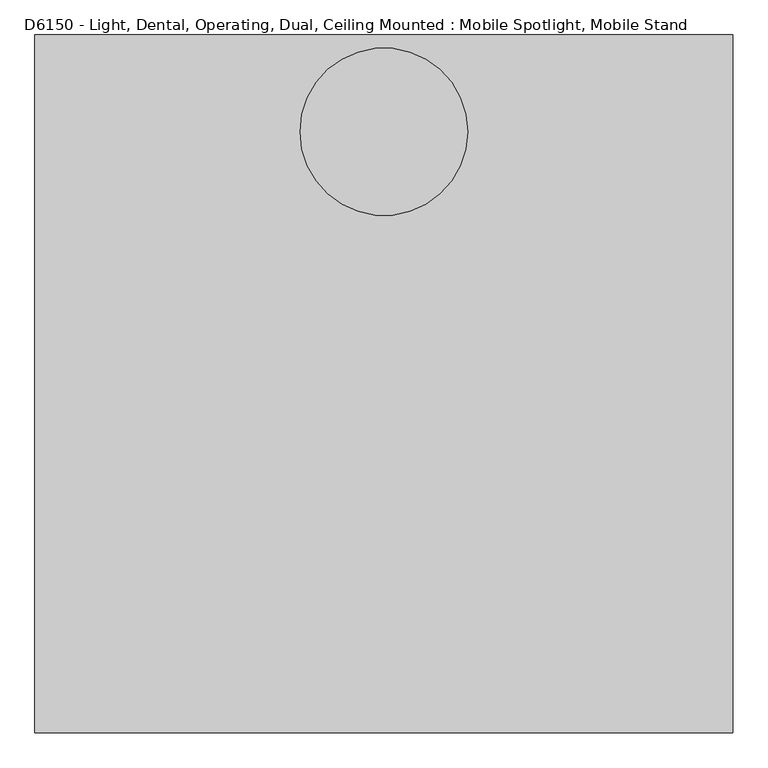
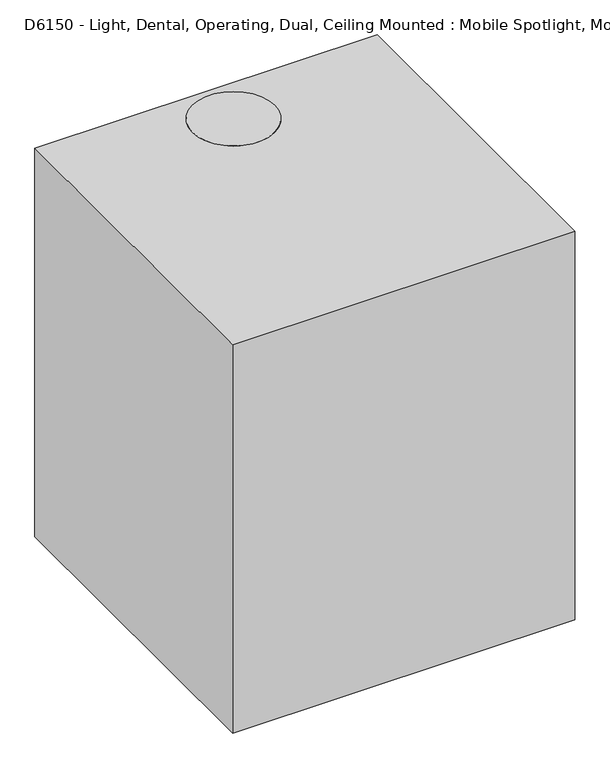
"""IFC4 building model written with IfcOpenShell, lengths in millimetres: proxy geometry, D6150 - Light, Dental, Operating, Dual, Ceiling Mounted : Mobile Spotlight, Mobile Stand."""

import ifcopenshell
import ifcopenshell.guid

model = None  # the IFC model being written
_history = None  # IfcOwnerHistory: only IFC2X3 demands one
_inside = {}  # id of a spatial element -> (the spatial element, [elements in it])
_under = {}  # id of a project, library or spatial element -> (it, [spatial elements below it])
_declared = {}  # id of a project -> (the project, [libraries it declares])
_typed = {}  # id of a type object -> (the type object, [elements of that type])
_made_of = {}  # id of a material, layer set ... -> (it, [elements and type objects made of it])


def new_model(schema):
    """Start an empty IFC model of exactly this schema.

    Asked for "IFC4X3", IfcOpenShell would pick the latest addendum, in which some entities
    have other attributes; the version numbers below select the first issue.
    IFC2X3 requires an IfcOwnerHistory on every rooted entity: one is made here for all.
    """
    global model, _history
    if schema == "IFC4X3":
        model = ifcopenshell.file(schema_version=(4, 3, 0, 0))
    else:
        model = ifcopenshell.file(schema=schema)
    _inside.clear()
    _under.clear()
    _declared.clear()
    _typed.clear()
    _made_of.clear()
    _history = None
    if model.schema == "IFC2X3":
        org = make("IfcOrganization", Name="unknown")
        user = make(
            "IfcPersonAndOrganization",
            ThePerson=make("IfcPerson", FamilyName="unknown"),
            TheOrganization=org,
        )
        app = make(
            "IfcApplication",
            ApplicationDeveloper=org,
            Version="unknown",
            ApplicationFullName="unknown",
            ApplicationIdentifier="unknown",
        )
        _history = make(
            "IfcOwnerHistory",
            OwningUser=user,
            OwningApplication=app,
            ChangeAction="ADDED",
            CreationDate=0,
        )
    return model


def make(cls, **values):
    """One entity of the class cls with the attributes given. An attribute that is None is left unset."""
    return model.create_entity(
        cls, **{name: value for name, value in values.items() if value is not None}
    )


def rooted(cls, **values):
    """An entity with a GlobalId (a new one), such as an element, a storey or a relation."""
    return make(cls, GlobalId=ifcopenshell.guid.new(), OwnerHistory=_history, **values)


def si_unit(unit_type, name, prefix=None):
    """IfcSIUnit, for example si_unit("LENGTHUNIT", "METRE", prefix="MILLI")."""
    return make("IfcSIUnit", UnitType=unit_type, Prefix=prefix, Name=name)


def assignment(units):
    """IfcUnitAssignment: the units of a project."""
    return None if units is None else make("IfcUnitAssignment", Units=units)


def point(xyz):
    """IfcCartesianPoint."""
    return None if xyz is None else make("IfcCartesianPoint", Coordinates=xyz)


def direction(xyz):
    """IfcDirection."""
    return None if xyz is None else make("IfcDirection", DirectionRatios=xyz)


def frame(location, z_axis=None, x_axis=None):
    """IfcAxis2Placement3D, a coordinate frame: its origin and axes. An axis left out is left unset."""
    return make(
        "IfcAxis2Placement3D",
        Location=point(location),
        Axis=direction(z_axis),
        RefDirection=direction(x_axis),
    )


def frame_2d(location, x_axis=None):
    """IfcAxis2Placement2D, a coordinate frame in the plane: its origin and x axis."""
    return make(
        "IfcAxis2Placement2D", Location=point(location), RefDirection=direction(x_axis)
    )


def origin():
    """The frame at (0, 0, 0) with its axes left unset."""
    return frame((0.0, 0.0, 0.0))


def place(relative_to, where):
    """IfcLocalPlacement: puts the frame where relative to a parent placement (None: the world)."""
    return make(
        "IfcLocalPlacement", PlacementRelTo=relative_to, RelativePlacement=where
    )


def context(
    kind, dimensions, precision=None, world=None, true_north=None, identifier=None
):
    """IfcGeometricRepresentationContext, for example the 3D "Model" context."""
    return make(
        "IfcGeometricRepresentationContext",
        ContextIdentifier=identifier,
        ContextType=kind,
        CoordinateSpaceDimension=dimensions,
        Precision=precision,
        WorldCoordinateSystem=world,
        TrueNorth=true_north,
    )


def project(units=None, contexts=None):
    """IfcProject with its units and contexts."""
    return rooted(
        "IfcProject",
        Name="project",
        RepresentationContexts=contexts,
        UnitsInContext=assignment(units),
    )


def spatial(cls, under=None, at=None, **own):
    """A site, building, storey or space (cls), placed at a placement, below another one or the project."""
    s = rooted(cls, ObjectPlacement=at, **own)
    if under is not None:
        _under.setdefault(under.id(), (under, []))[1].append(s)
    return s


def polyline(points):
    """IfcPolyline through the points."""
    return make("IfcPolyline", Points=[point(p) for p in points])


def circle_curve(where, radius):
    """IfcCircle in the frame where."""
    return make("IfcCircle", Position=where, Radius=radius)


def ellipse_curve(where, semi_axis1, semi_axis2):
    """IfcEllipse in the frame where."""
    return make(
        "IfcEllipse", Position=where, SemiAxis1=semi_axis1, SemiAxis2=semi_axis2
    )


def trimmed(basis, trim1, trim2, sense, master):
    """IfcTrimmedCurve: the piece of a basis curve between two trims."""
    return make(
        "IfcTrimmedCurve",
        BasisCurve=basis,
        Trim1=trim1,
        Trim2=trim2,
        SenseAgreement=sense,
        MasterRepresentation=master,
    )


def segment(curve, same_sense, transition):
    """IfcCompositeCurveSegment."""
    return make(
        "IfcCompositeCurveSegment",
        Transition=transition,
        SameSense=same_sense,
        ParentCurve=curve,
    )


def composite_curve(segments, self_intersect=None):
    """IfcCompositeCurve: segments joined end to end."""
    return make("IfcCompositeCurve", Segments=segments, SelfIntersect=self_intersect)


def outline(outer, holes=None, kind="AREA"):
    """IfcArbitraryClosedProfileDef: a profile drawn as a closed curve; with holes, ...WithVoids."""
    if holes is None:
        return make("IfcArbitraryClosedProfileDef", ProfileType=kind, OuterCurve=outer)
    return make(
        "IfcArbitraryProfileDefWithVoids",
        ProfileType=kind,
        OuterCurve=outer,
        InnerCurves=holes,
    )


def extrude(swept, where, along, depth):
    """IfcExtrudedAreaSolid: the profile swept, set in the frame where, extruded along a direction by depth."""
    return make(
        "IfcExtrudedAreaSolid",
        SweptArea=swept,
        Position=where,
        ExtrudedDirection=direction(along),
        Depth=depth,
    )


def shape(context_of_items, identifier, shape_type, items):
    """IfcShapeRepresentation: the items that make up one representation, for example the "Body"."""
    return make(
        "IfcShapeRepresentation",
        ContextOfItems=context_of_items,
        RepresentationIdentifier=identifier,
        RepresentationType=shape_type,
        Items=items,
    )


def source(mapping_origin, context_of_items, identifier, shape_type, items):
    """IfcRepresentationMap: a shape defined once, which mapped items show again and again."""
    return make(
        "IfcRepresentationMap",
        MappingOrigin=mapping_origin,
        MappedRepresentation=shape(context_of_items, identifier, shape_type, items),
    )


def transform(
    local_origin,
    x_axis=None,
    y_axis=None,
    z_axis=None,
    scale=None,
    scale2=None,
    scale3=None,
    uniform=True,
):
    """IfcCartesianTransformationOperator3D, or its non-uniform kind. x_axis, y_axis, z_axis: its Axis1, 2, 3."""
    if uniform:
        return make(
            "IfcCartesianTransformationOperator3D",
            Axis1=direction(x_axis),
            Axis2=direction(y_axis),
            LocalOrigin=point(local_origin),
            Scale=scale,
            Axis3=direction(z_axis),
        )
    return make(
        "IfcCartesianTransformationOperator3DnonUniform",
        Axis1=direction(x_axis),
        Axis2=direction(y_axis),
        LocalOrigin=point(local_origin),
        Scale=scale,
        Axis3=direction(z_axis),
        Scale2=scale2,
        Scale3=scale3,
    )


def mapped(mapping_source, mapping_target):
    """IfcMappedItem: shows the shape of a source again, moved by a transform."""
    return make(
        "IfcMappedItem", MappingSource=mapping_source, MappingTarget=mapping_target
    )


def made_of(thing, what):
    """Note that an element or type object is made of a material, layer set ...; save() writes the relation."""
    if what is not None:
        _made_of.setdefault(what.id(), (what, []))[1].append(thing)
    return thing


def element(
    cls,
    number,
    at=None,
    inside=None,
    cuts=None,
    type_object=None,
    material=None,
    context=None,
    identifier="Body",
    shape_type=None,
    held_by="IfcProductDefinitionShape",
    body=None,
    shapes=None,
    **own,
):
    """One element of the class cls, such as IfcWall. Its Tag is "e" and its number.

    at: its placement. inside: the storey or other place that contains it. cuts: it is an
    opening in that element (IfcRelVoidsElement). A single representation is given by context,
    identifier, shape_type and body (its items); several are given by shapes. held_by: the class
    of the entity that holds the representations. save() writes the other relations.
    """
    e = rooted(cls, Tag="e%d" % number, ObjectPlacement=at, **own)
    if body is not None:
        shapes = [shape(context, identifier, shape_type, body)]
    if shapes is not None:
        e.Representation = make(held_by, Representations=shapes)
    if inside is not None:
        _inside.setdefault(inside.id(), (inside, []))[1].append(e)
    if cuts is not None:
        rooted(
            "IfcRelVoidsElement", RelatingBuildingElement=cuts, RelatedOpeningElement=e
        )
    if type_object is not None:
        _typed.setdefault(type_object.id(), (type_object, []))[1].append(e)
    return made_of(e, material)


def aggregate(whole, parts):
    """IfcRelAggregates: a whole, such as a stair, and the parts it consists of."""
    return rooted("IfcRelAggregates", RelatingObject=whole, RelatedObjects=parts)


def save(model, path):
    """Write the relations noted so far, then the file.

    IfcRelAggregates (storeys below a building ...), IfcRelContainedInSpatialStructure (elements
    in a storey), IfcRelDefinesByType, IfcRelAssociatesMaterial and IfcRelDeclares: one each for
    every whole, place, type object, material and project.
    """
    for whole, parts in _under.values():
        aggregate(whole, parts)
    for where, things in _inside.values():
        rooted(
            "IfcRelContainedInSpatialStructure",
            RelatedElements=things,
            RelatingStructure=where,
        )
    for kind, things in _typed.values():
        rooted("IfcRelDefinesByType", RelatedObjects=things, RelatingType=kind)
    for what, things in _made_of.values():
        rooted("IfcRelAssociatesMaterial", RelatedObjects=things, RelatingMaterial=what)
    for by, libraries in _declared.values():
        rooted("IfcRelDeclares", RelatingContext=by, RelatedDefinitions=libraries)
    model.write(path)


def plane_surface(at):
    """IfcPlane: the flat surface through the origin of the frame at, square to its z axis."""
    return make("IfcPlane", Position=at)


def revolved_surface(curve, axis_point, axis_direction):
    """IfcSurfaceOfRevolution: the curve turned about the line through axis_point along axis_direction."""
    return make(
        "IfcSurfaceOfRevolution",
        SweptCurve=make("IfcArbitraryOpenProfileDef", ProfileType="CURVE", Curve=curve),
        AxisPosition=make("IfcAxis1Placement", Location=point(axis_point), Axis=direction(axis_direction)),
    )


def advanced_brep(points, edges, surfaces, faces):
    """IfcAdvancedBrep: a solid bounded by faces that lie on surfaces and meet in shared edges.

    An edge is (start, end): straight between two places in points (the first is 0);
    or (start, end, curve); or (start, end, curve, False) where it runs against its curve.
    A face is (place in surfaces, loops), or (place, loops, False) where it looks against
    its surface's normal. A loop lists edges by number (the first is 1), with a minus sign
    where the edge is run from its end to its start. The first loop is the outer one.
    """
    corners = [point(p) for p in points]
    vertices = [make("IfcVertexPoint", VertexGeometry=c) for c in corners]
    made = []
    for start, end, *more in edges:
        made.append(
            make(
                "IfcEdgeCurve",
                EdgeStart=vertices[start],
                EdgeEnd=vertices[end],
                EdgeGeometry=more[0] if more else make("IfcPolyline", Points=[corners[start], corners[end]]),
                SameSense=more[1] if len(more) > 1 else True,
            )
        )
    hull = []
    for where, loops, *sense in faces:
        bounds = []
        for j, loop in enumerate(loops):
            ring = [make("IfcOrientedEdge", EdgeElement=made[abs(k) - 1], Orientation=k > 0) for k in loop]
            bounds.append(
                make(
                    "IfcFaceOuterBound" if j == 0 else "IfcFaceBound",
                    Bound=make("IfcEdgeLoop", EdgeList=ring),
                    Orientation=True,
                )
            )
        hull.append(make("IfcAdvancedFace", Bounds=bounds, FaceSurface=surfaces[where], SameSense=sense[0] if sense else True))
    return make("IfcAdvancedBrep", Outer=make("IfcClosedShell", CfsFaces=hull))


def d6150_light_dental_operating_dual_ceiling_mounted_mobile_95434ab8(model_context):
    return source(origin(), model_context, "Body", "SolidModel", [
        extrude(outline(composite_curve([segment(polyline([(-39.1500071, -1119.0842165), (-39.1500071, -653.3774924)]), True, "CONTINUOUS"), segment(trimmed(circle_curve(frame_2d((-20.1000071, -639.2363382)), 23.7249814), [point((-39.1500071, -653.3774924))], [point((-1.0500071, -653.3774924))], True, "CARTESIAN"), True, "CONTINUOUS"), segment(polyline([(-1.0500071, -653.3774924), (-1.0500071, -1119.0842165), (-39.1500071, -1119.0842165)]), True, "CONTINUOUS")], self_intersect=False)), frame((393.4202731, 0.0, 0.0), z_axis=(1.0, 0.0, 0.0), x_axis=(0.0, 1.0, 0.0)), (0.0, 0.0, 1.0), 44.7313138),
        extrude(outline(composite_curve([segment(trimmed(circle_curve(frame_2d((73.025, 3.175)), 3.175), [point((73.025, 0.0))], [point((76.2, 3.175))], True, "CARTESIAN"), True, "CONTINUOUS"), segment(polyline([(76.2, 3.175), (76.2, 34.925)]), True, "CONTINUOUS"), segment(trimmed(circle_curve(frame_2d((79.375, 34.925)), 3.175), [point((76.2, 34.925))], [point((79.375, 38.1))], False, "CARTESIAN"), True, "CONTINUOUS"), segment(trimmed(circle_curve(frame_2d((79.375, 34.925)), 3.175), [point((79.375, 38.1))], [point((82.55, 34.925))], False, "CARTESIAN"), True, "CONTINUOUS"), segment(polyline([(82.55, 34.925), (82.55, -41.275)]), True, "CONTINUOUS"), segment(trimmed(circle_curve(frame_2d((79.375, -41.275)), 3.175), [point((82.55, -41.275))], [point((79.375, -44.4499999))], False, "CARTESIAN"), True, "CONTINUOUS"), segment(trimmed(circle_curve(frame_2d((79.375, -41.275)), 3.175), [point((79.375, -44.4499999))], [point((76.2, -41.275))], False, "CARTESIAN"), True, "CONTINUOUS"), segment(polyline([(76.2, -41.275), (76.2, -9.525)]), True, "CONTINUOUS"), segment(trimmed(circle_curve(frame_2d((73.025, -9.525)), 3.175), [point((76.2, -9.525))], [point((73.025, -6.35))], True, "CARTESIAN"), True, "CONTINUOUS"), segment(polyline([(73.025, -6.35), (-6.35, -6.35), (-6.35, 0.0), (73.025, 0.0)]), True, "CONTINUOUS")], self_intersect=False)), frame((542.925, -72.7377417, -1373.8729915), z_axis=(0.0, -0.3420201433256747, 0.9396926207859062), x_axis=(1.0, 0.0, 0.0)), (0.0, 0.0, 1.0), 6.35),
        extrude(outline(composite_curve([segment(polyline([(3.175, 3.175), (3.175, 82.55), (9.525, 82.55), (9.525, 3.175)]), True, "CONTINUOUS"), segment(trimmed(circle_curve(frame_2d((12.7, 3.175)), 3.175), [point((9.525, 3.175))], [point((12.7, 0.0))], True, "CARTESIAN"), True, "CONTINUOUS"), segment(polyline([(12.7, 0.0), (44.45, 0.0)]), True, "CONTINUOUS"), segment(trimmed(circle_curve(frame_2d((44.45, -3.175)), 3.175), [point((44.45, 0.0))], [point((47.6249999, -3.175))], False, "CARTESIAN"), True, "CONTINUOUS"), segment(trimmed(circle_curve(frame_2d((44.45, -3.175)), 3.175), [point((47.6249999, -3.175))], [point((44.45, -6.35))], False, "CARTESIAN"), True, "CONTINUOUS"), segment(polyline([(44.45, -6.35), (-31.75, -6.35)]), True, "CONTINUOUS"), segment(trimmed(circle_curve(frame_2d((-31.75, -3.175)), 3.175), [point((-31.75, -6.35))], [point((-34.925, -3.175))], False, "CARTESIAN"), True, "CONTINUOUS"), segment(trimmed(circle_curve(frame_2d((-31.75, -3.175)), 3.175), [point((-34.925, -3.175))], [point((-31.75, 0.0))], False, "CARTESIAN"), True, "CONTINUOUS"), segment(polyline([(-31.75, 0.0), (0.0, 0.0)]), True, "CONTINUOUS"), segment(trimmed(circle_curve(frame_2d((0.0, 3.175)), 3.175), [point((0.0, 0.0))], [point((3.175, 3.175))], True, "CARTESIAN"), True, "CONTINUOUS")], self_intersect=False)), frame((193.675, -69.7542176, -1372.7870776), z_axis=(0.0, -0.3420201433256747, 0.9396926207859062), x_axis=(0.0, -0.9396926207859062, -0.3420201433256747)), (0.0, 0.0, 1.0), 6.35),
        extrude(outline(polyline([(0.0, 0.0), (82.4409767, 0.0), (82.4409767, 239.4711286), (0.0, 239.4711286), (0.0, 249.9105643), (93.5534767, 249.9105643), (93.5534767, -10.4394357), (0.0, -10.4394357), (0.0, 0.0)])), frame((526.1355643, -133.3040801, -1296.3598055), z_axis=(0.0, 0.9396926207859063, 0.3420201433256747), x_axis=(0.0, 0.3420201433256747, -0.9396926207859063)), (0.0, 0.0, 1.0), 51.6611993),
        extrude(outline(composite_curve([segment(polyline([(86.8443674, -1273.5552985), (50.1090556, -1317.3347385), (-223.5123411, -1416.9247823), (-279.7941042, -1407.0007889)]), True, "CONTINUOUS"), segment(trimmed(circle_curve(frame_2d((-47.9034041, -1473.7270449)), 241.3), [point((-279.7941042, -1407.0007889))], [point((86.8443674, -1273.5552985))], False, "CARTESIAN"), True, "CONTINUOUS")], self_intersect=False)), frame((286.6644357, 0.0, 0.0), z_axis=(1.0, 0.0, 0.0), x_axis=(0.0, 1.0, 0.0)), (0.0, 0.0, 1.0), 239.4711286),
        extrude(outline(composite_curve([segment(trimmed(circle_curve(frame_2d((-46.1031431, -1478.6732215)), 259.8923153), [point((-297.6952486, -1413.5162727))], [point((104.7455119, -1267.0398148))], False, "CARTESIAN"), True, "CONTINUOUS"), segment(polyline([(104.7455119, -1267.0398148), (86.8443674, -1273.5552985)]), True, "CONTINUOUS"), segment(trimmed(circle_curve(frame_2d((-47.9034041, -1473.7270449)), 241.3), [point((86.8443674, -1273.5552985))], [point((-279.7941042, -1407.0007889))], True, "CARTESIAN"), True, "CONTINUOUS"), segment(polyline([(-279.7941042, -1407.0007889), (-297.6952486, -1413.5162727)]), True, "CONTINUOUS")], self_intersect=False)), frame((286.6644357, 0.0, 0.0), z_axis=(1.0, 0.0, 0.0), x_axis=(0.0, 1.0, 0.0)), (0.0, 0.0, 1.0), 239.4711286),
        extrude(outline(polyline([(-94.9611341, -1311.6988489), (-86.5874476, -1314.7466215), (-85.0400529, -1323.5223329), (-91.8663446, -1329.2502718), (-100.2400311, -1326.2024992), (-101.7874258, -1317.4267877), (-94.9611341, -1311.6988489)])), frame((269.875, 0.0, 0.0), z_axis=(1.0, 0.0, 0.0), x_axis=(0.0, 1.0, 0.0)), (0.0, 0.0, 1.0), 3.175),
        extrude(outline(composite_curve([segment(trimmed(circle_curve(frame_2d((-94.5189227, -1319.4941842)), 25.4), [point((-69.1189227, -1319.4941842))], [point((-119.9189227, -1319.4941842))], False, "CARTESIAN"), True, "CONTINUOUS"), segment(trimmed(circle_curve(frame_2d((-94.5189227, -1319.4941842)), 25.4), [point((-119.9189227, -1319.4941842))], [point((-69.1189227, -1319.4941842))], False, "CARTESIAN"), True, "CONTINUOUS")], self_intersect=False)), frame((276.225, 0.0, 0.0), z_axis=(1.0, 0.0, 0.0), x_axis=(0.0, 1.0, 0.0)), (0.0, 0.0, 1.0), 10.4394357),
        extrude(outline(composite_curve([segment(polyline([(-3.4680197, -1125.1377649), (-78.542022, -1331.4018912)]), True, "CONTINUOUS"), segment(trimmed(circle_curve(frame_2d((-96.5270837, -1321.9059271)), 20.3380376), [point((-78.542022, -1331.4018912))], [point((-116.6187215, -1318.7496851))], False, "CARTESIAN"), True, "CONTINUOUS"), segment(polyline([(-116.6187215, -1318.7496851), (-43.9924341, -1119.2106004)]), True, "CONTINUOUS"), segment(trimmed(circle_curve(frame_2d((-36.2019563, -1122.0461024)), 8.2904533), [point((-43.9924341, -1119.2106004))], [point((-33.3664543, -1114.2556246))], False, "CARTESIAN"), True, "CONTINUOUS"), segment(polyline([(-33.3664543, -1114.2556246), (-3.4680197, -1125.1377649)]), True, "CONTINUOUS")], self_intersect=False), holes=[composite_curve([segment(trimmed(circle_curve(frame_2d((-93.7032837, -1319.6305836)), 4.6125063), [point((-89.0907774, -1319.6305836))], [point((-98.31579, -1319.6305836))], True, "CARTESIAN"), True, "CONTINUOUS"), segment(trimmed(circle_curve(frame_2d((-93.7032837, -1319.6305836)), 4.6125063), [point((-98.31579, -1319.6305836))], [point((-89.0907774, -1319.6305836))], True, "CARTESIAN"), True, "CONTINUOUS")], self_intersect=False)]), frame((273.05, 0.0, 0.0), z_axis=(1.0, 0.0, 0.0), x_axis=(0.0, 1.0, 0.0)), (0.0, 0.0, 1.0), 3.175),
        extrude(outline(polyline([(-94.9611341, -1311.6988489), (-86.5874476, -1314.7466215), (-85.0400529, -1323.5223329), (-91.8663446, -1329.2502718), (-100.2400311, -1326.2024992), (-101.7874258, -1317.4267877), (-94.9611341, -1311.6988489)])), frame((539.75, 0.0, 0.0), z_axis=(1.0, 0.0, 0.0), x_axis=(0.0, 1.0, 0.0)), (0.0, 0.0, 1.0), 3.175),
        extrude(outline(composite_curve([segment(polyline([(-3.4680197, -1125.1377649), (-14.3271592, -1154.9730056), (-52.0160716, -1141.2553633), (-44.2468396, -1119.9095738)]), True, "CONTINUOUS"), segment(trimmed(circle_curve(frame_2d((-35.7573884, -1122.9994814)), 9.0342853), [point((-44.2468396, -1119.9095738))], [point((-32.6674808, -1114.5100302))], False, "CARTESIAN"), True, "CONTINUOUS"), segment(polyline([(-32.6674808, -1114.5100302), (-3.4680197, -1125.1377649)]), True, "CONTINUOUS")], self_intersect=False)), frame((276.225, 0.0, 0.0), z_axis=(1.0, 0.0, 0.0), x_axis=(0.0, 1.0, 0.0)), (0.0, 0.0, 1.0), 260.35),
        extrude(outline(composite_curve([segment(trimmed(circle_curve(frame_2d((-94.5189227, -1319.4941842)), 25.4), [point((-69.1189227, -1319.4941842))], [point((-119.9189227, -1319.4941842))], False, "CARTESIAN"), True, "CONTINUOUS"), segment(trimmed(circle_curve(frame_2d((-94.5189227, -1319.4941842)), 25.4), [point((-119.9189227, -1319.4941842))], [point((-69.1189227, -1319.4941842))], False, "CARTESIAN"), True, "CONTINUOUS")], self_intersect=False)), frame((526.1355643, 0.0, 0.0), z_axis=(1.0, 0.0, 0.0), x_axis=(0.0, 1.0, 0.0)), (0.0, 0.0, 1.0), 10.4394357),
        extrude(outline(composite_curve([segment(polyline([(-3.4680197, -1125.1377649), (-78.542022, -1331.4018912)]), True, "CONTINUOUS"), segment(trimmed(circle_curve(frame_2d((-96.5270837, -1321.9059271)), 20.3380376), [point((-78.542022, -1331.4018912))], [point((-116.6187215, -1318.7496851))], False, "CARTESIAN"), True, "CONTINUOUS"), segment(polyline([(-116.6187215, -1318.7496851), (-43.9252942, -1119.026135)]), True, "CONTINUOUS"), segment(trimmed(circle_curve(frame_2d((-36.3192818, -1121.7944972)), 8.0941494), [point((-43.9252942, -1119.026135))], [point((-33.5509196, -1114.1884847))], False, "CARTESIAN"), True, "CONTINUOUS"), segment(polyline([(-33.5509196, -1114.1884847), (-3.4680197, -1125.1377649)]), True, "CONTINUOUS")], self_intersect=False), holes=[composite_curve([segment(trimmed(circle_curve(frame_2d((-93.7032837, -1319.6305836)), 4.6125063), [point((-89.0907774, -1319.6305836))], [point((-98.31579, -1319.6305836))], True, "CARTESIAN"), True, "CONTINUOUS"), segment(trimmed(circle_curve(frame_2d((-93.7032837, -1319.6305836)), 4.6125063), [point((-98.31579, -1319.6305836))], [point((-89.0907774, -1319.6305836))], True, "CARTESIAN"), True, "CONTINUOUS")], self_intersect=False)]), frame((536.575, 0.0, 0.0), z_axis=(1.0, 0.0, 0.0), x_axis=(0.0, 1.0, 0.0)), (0.0, 0.0, 1.0), 3.175),
        extrude(outline(composite_curve([segment(polyline([(2.3510297, -624.5764556), (2.3510297, -647.2535292)]), True, "CONTINUOUS"), segment(trimmed(circle_curve(frame_2d((-19.8739703, -638.9514742)), 23.7249814), [point((2.3510297, -647.2535292))], [point((-42.0989703, -647.2535292))], False, "CARTESIAN"), True, "CONTINUOUS"), segment(polyline([(-42.0989703, -647.2535292), (-42.0989703, -624.5764556)]), True, "CONTINUOUS"), segment(trimmed(circle_curve(frame_2d((-19.8739703, -632.8785107)), 23.7249814), [point((-42.0989703, -624.5764556))], [point((2.3510297, -624.5764556))], False, "CARTESIAN"), True, "CONTINUOUS")], self_intersect=False)), frame((387.35, 0.0, 0.0), z_axis=(1.0, 0.0, 0.0), x_axis=(0.0, 1.0, 0.0)), (0.0, 0.0, 1.0), 56.9609543),
        extrude(outline(composite_curve([segment(polyline([(435.4536657, -616.8649924), (454.2128177, -627.6955939), (454.2128177, -644.134391), (435.4536657, -654.9649924), (-2.6963343, -654.9649924)]), True, "CONTINUOUS"), segment(trimmed(circle_curve(frame_2d((-16.8374885, -635.9149924)), 23.7249814), [point((-2.6963343, -654.9649924))], [point((-2.6963343, -616.8649924))], True, "CARTESIAN"), True, "CONTINUOUS"), segment(polyline([(-2.6963343, -616.8649924), (435.4536657, -616.8649924)]), True, "CONTINUOUS")], self_intersect=False)), frame((393.4202731, 0.0, 0.0), z_axis=(1.0, 0.0, 0.0), x_axis=(0.0, 1.0, 0.0)), (0.0, 0.0, 1.0), 44.7313138),
        advanced_brep(
        [(415.78593, 503.9195844, -657.1847366), (415.78593, 458.5654372, -657.1847366), (415.78593, 481.2425108, -657.1847366), (415.78593, 481.2425108, -612.7347366), (415.78593, 458.5654372, -612.7347366), (415.78593, 503.9195844, -612.7347366)],
        [
            (0, 1, circle_curve(frame((415.78593, 481.2425108, -657.1847366), z_axis=(0.0, 0.0, -1.0), x_axis=(0.0, -1.0, 0.0)), 22.6770736)),
            (1, 2),
            (2, 0),
            (1, 0, circle_curve(frame((415.78593, 481.2425108, -657.1847366), z_axis=(0.0, 0.0, -1.0), x_axis=(0.0, -1.0, 0.0)), 22.6770736)),
            (3, 4),
            (4, 5, circle_curve(frame((415.78593, 481.2425108, -612.7347366), z_axis=(0.0, 0.0, 1.0), x_axis=(0.0, -1.0, 0.0)), 22.6770736)),
            (5, 3),
            (5, 4, circle_curve(frame((415.78593, 481.2425108, -612.7347366), z_axis=(0.0, 0.0, 1.0), x_axis=(0.0, -1.0, 0.0)), 22.6770736)),
            (4, 1, circle_curve(frame((415.78593, 466.8674922, -634.9597366), z_axis=(1.0, 0.0, 0.0), x_axis=(0.0, 1.0, 0.0)), 23.7249814)),
            (0, 5, circle_curve(frame((415.78593, 495.6175294, -634.9597366), z_axis=(1.0, 0.0, 0.0), x_axis=(0.0, -1.0, 0.0)), 23.7249814)),
        ],
        [
            plane_surface(frame((415.78593, 481.2425108, -657.1847366), z_axis=(0.0, 0.0, -1.0), x_axis=(0.0, -1.0, 0.0))),
            plane_surface(frame((415.78593, 481.2425108, -612.7347366), z_axis=(0.0, 0.0, 1.0), x_axis=(0.0, -1.0, 0.0))),
            revolved_surface(trimmed(ellipse_curve(frame((415.78593, 466.8674922, -634.9597366), z_axis=(-1.0, 0.0, 0.0), x_axis=(0.0, 1.0, 0.0)), 23.7249814, 23.7249814), [point((415.78593, 458.5654372, -657.1847366))], [point((415.78593, 458.5654372, -612.7347366))], True, "CARTESIAN"), (415.78593, 481.2425108, -657.1847366), (0.0, 0.0, 1.0)),
        ],
        [
            (0, [[1, 2, 3]]),
            (0, [[4, -3, -2]]),
            (1, [[5, 6, 7]]),
            (1, [[-7, 8, -5]]),
            (2, [[-6, 9, -1, 10]]),
            (2, [[-8, -10, -4, -9]]),
        ],
    ),
        extrude(outline(composite_curve([segment(trimmed(circle_curve(frame_2d((479.6550108, -634.9597366)), 19.05), [point((460.6050108, -634.9597366))], [point((498.7050108, -634.9597366))], False, "CARTESIAN"), True, "CONTINUOUS"), segment(trimmed(circle_curve(frame_2d((479.6550108, -634.9597366)), 19.05), [point((498.7050108, -634.9597366))], [point((460.6050108, -634.9597366))], False, "CARTESIAN"), True, "CONTINUOUS")], self_intersect=False)), frame((88.6202731, 0.0, 0.0), z_axis=(1.0, 0.0, 0.0), x_axis=(0.0, 1.0, 0.0)), (0.0, 0.0, 1.0), 304.8),
        extrude(outline(composite_curve([segment(trimmed(circle_curve(frame_2d((479.6550108, -634.9597366)), 22.225), [point((501.8800108, -634.9597366))], [point((457.4300108, -634.9597366))], False, "CARTESIAN"), True, "CONTINUOUS"), segment(trimmed(circle_curve(frame_2d((479.6550108, -634.9597366)), 22.225), [point((457.4300108, -634.9597366))], [point((501.8800108, -634.9597366))], False, "CARTESIAN"), True, "CONTINUOUS")], self_intersect=False)), frame((50.968278, 0.0, 0.0), z_axis=(1.0, 0.0, 0.0), x_axis=(0.0, 1.0, 0.0)), (0.0, 0.0, 1.0), 37.6519951),
        extrude(outline(composite_curve([segment(polyline([(-42.2464852, -1119.0842165), (-42.2464852, -653.3774924)]), True, "CONTINUOUS"), segment(trimmed(circle_curve(frame_2d((-23.1964852, -639.2363382)), 23.7249814), [point((-42.2464852, -653.3774924))], [point((-4.1464852, -653.3774924))], True, "CARTESIAN"), True, "CONTINUOUS"), segment(polyline([(-4.1464852, -653.3774924), (-4.1464852, -1119.0842165), (-42.2464852, -1119.0842165)]), True, "CONTINUOUS")], self_intersect=False)), frame((-438.1515869, 0.0, 0.0), z_axis=(1.0, 0.0, 0.0), x_axis=(0.0, 1.0, 0.0)), (0.0, 0.0, 1.0), 44.7313138),
        extrude(outline(composite_curve([segment(polyline([(3.1749999, 3.175), (3.1749999, 82.55), (9.525, 82.55), (9.525, 3.175)]), True, "CONTINUOUS"), segment(trimmed(circle_curve(frame_2d((12.6999999, 3.175)), 3.175), [point((9.525, 3.175))], [point((12.6999999, 0.0))], True, "CARTESIAN"), True, "CONTINUOUS"), segment(polyline([(12.6999999, 0.0), (44.45, 0.0)]), True, "CONTINUOUS"), segment(trimmed(circle_curve(frame_2d((44.45, -3.175)), 3.175), [point((44.45, 0.0))], [point((47.6249999, -3.175))], False, "CARTESIAN"), True, "CONTINUOUS"), segment(trimmed(circle_curve(frame_2d((44.45, -3.175)), 3.175), [point((47.6249999, -3.175))], [point((44.45, -6.35))], False, "CARTESIAN"), True, "CONTINUOUS"), segment(polyline([(44.45, -6.35), (-31.75, -6.35)]), True, "CONTINUOUS"), segment(trimmed(circle_curve(frame_2d((-31.75, -3.175)), 3.175), [point((-31.75, -6.35))], [point((-34.925, -3.175))], False, "CARTESIAN"), True, "CONTINUOUS"), segment(trimmed(circle_curve(frame_2d((-31.75, -3.175)), 3.175), [point((-34.925, -3.175))], [point((-31.75, 0.0))], False, "CARTESIAN"), True, "CONTINUOUS"), segment(polyline([(-31.75, 0.0), (0.0, 0.0)]), True, "CONTINUOUS"), segment(trimmed(circle_curve(frame_2d((0.0, 3.175)), 3.175), [point((0.0, 0.0))], [point((3.1749999, 3.175))], True, "CARTESIAN"), True, "CONTINUOUS")], self_intersect=False)), frame((-619.125, -72.8506957, -1372.7870776), z_axis=(0.0, -0.3420201433256747, 0.9396926207859062), x_axis=(0.0, -0.9396926207859062, -0.3420201433256747)), (0.0, 0.0, 1.0), 6.35),
        extrude(outline(composite_curve([segment(trimmed(circle_curve(frame_2d((73.025, 3.1749999)), 3.175), [point((73.025, 0.0))], [point((76.2, 3.1749999))], True, "CARTESIAN"), True, "CONTINUOUS"), segment(polyline([(76.2, 3.1749999), (76.2, 34.9249999)]), True, "CONTINUOUS"), segment(trimmed(circle_curve(frame_2d((79.375, 34.9249999)), 3.175), [point((76.2, 34.9249999))], [point((79.375, 38.0999999))], False, "CARTESIAN"), True, "CONTINUOUS"), segment(trimmed(circle_curve(frame_2d((79.375, 34.9249999)), 3.175), [point((79.375, 38.0999999))], [point((82.55, 34.9249999))], False, "CARTESIAN"), True, "CONTINUOUS"), segment(polyline([(82.55, 34.9249999), (82.55, -41.2750001)]), True, "CONTINUOUS"), segment(trimmed(circle_curve(frame_2d((79.375, -41.2750001)), 3.175), [point((82.55, -41.2750001))], [point((79.375, -44.45))], False, "CARTESIAN"), True, "CONTINUOUS"), segment(trimmed(circle_curve(frame_2d((79.375, -41.2750001)), 3.175), [point((79.375, -44.45))], [point((76.2, -41.2750001))], False, "CARTESIAN"), True, "CONTINUOUS"), segment(polyline([(76.2, -41.2750001), (76.2, -9.525)]), True, "CONTINUOUS"), segment(trimmed(circle_curve(frame_2d((73.025, -9.525)), 3.175), [point((76.2, -9.525))], [point((73.025, -6.3500001))], True, "CARTESIAN"), True, "CONTINUOUS"), segment(polyline([(73.025, -6.3500001), (-6.35, -6.3500001), (-6.35, 0.0), (73.025, 0.0)]), True, "CONTINUOUS")], self_intersect=False)), frame((-269.875, -75.8342197, -1373.8729915), z_axis=(0.0, -0.3420201433256747, 0.9396926207859062), x_axis=(1.0, 0.0, 0.0)), (0.0, 0.0, 1.0), 6.35),
        extrude(outline(polyline([(-10.4394357, 0.0), (0.0, 0.0), (0.0, -93.5534767), (-260.35, -93.5534767), (-260.35, 0.0), (-249.9105643, 0.0), (-249.9105643, -82.4409766), (-10.4394357, -82.4409766), (-10.4394357, 0.0)])), frame((-536.575, -136.4005581, -1296.3598055), z_axis=(0.0, 0.9396926207859062, 0.34202014332567465), x_axis=(-1.0, 0.0, 0.0)), (0.0, 0.0, 1.0), 51.6611993),
        extrude(outline(composite_curve([segment(polyline([(83.7478894, -1273.5552985), (47.0125775, -1317.3347385), (-226.6088192, -1416.9247823), (-282.8905822, -1407.0007889)]), True, "CONTINUOUS"), segment(trimmed(circle_curve(frame_2d((-50.9998822, -1473.7270449)), 241.3), [point((-282.8905822, -1407.0007889))], [point((83.7478894, -1273.5552985))], False, "CARTESIAN"), True, "CONTINUOUS")], self_intersect=False)), frame((-526.1355643, 0.0, 0.0), z_axis=(1.0, 0.0, 0.0), x_axis=(0.0, 1.0, 0.0)), (0.0, 0.0, 1.0), 239.4711286),
        extrude(outline(composite_curve([segment(trimmed(circle_curve(frame_2d((-49.1996212, -1478.6732215)), 259.8923153), [point((-300.7917267, -1413.5162727))], [point((101.6490338, -1267.0398148))], False, "CARTESIAN"), True, "CONTINUOUS"), segment(polyline([(101.6490338, -1267.0398148), (83.7478894, -1273.5552985)]), True, "CONTINUOUS"), segment(trimmed(circle_curve(frame_2d((-50.9998822, -1473.7270449)), 241.3), [point((83.7478894, -1273.5552985))], [point((-282.8905822, -1407.0007889))], True, "CARTESIAN"), True, "CONTINUOUS"), segment(polyline([(-282.8905822, -1407.0007889), (-300.7917267, -1413.5162727)]), True, "CONTINUOUS")], self_intersect=False)), frame((-526.1355643, 0.0, 0.0), z_axis=(1.0, 0.0, 0.0), x_axis=(0.0, 1.0, 0.0)), (0.0, 0.0, 1.0), 239.4711286),
        extrude(outline(polyline([(-98.0576121, -1311.6988489), (-89.6839257, -1314.7466215), (-88.136531, -1323.5223329), (-94.9628227, -1329.2502718), (-103.3365092, -1326.2024992), (-104.8839039, -1317.4267877), (-98.0576121, -1311.6988489)])), frame((-273.05, 0.0, 0.0), z_axis=(1.0, 0.0, 0.0), x_axis=(0.0, 1.0, 0.0)), (0.0, 0.0, 1.0), 3.175),
        extrude(outline(composite_curve([segment(trimmed(circle_curve(frame_2d((-97.6154008, -1319.4941842)), 25.4), [point((-72.2154008, -1319.4941842))], [point((-123.0154008, -1319.4941842))], False, "CARTESIAN"), True, "CONTINUOUS"), segment(trimmed(circle_curve(frame_2d((-97.6154008, -1319.4941842)), 25.4), [point((-123.0154008, -1319.4941842))], [point((-72.2154008, -1319.4941842))], False, "CARTESIAN"), True, "CONTINUOUS")], self_intersect=False)), frame((-286.6644357, 0.0, 0.0), z_axis=(1.0, 0.0, 0.0), x_axis=(0.0, 1.0, 0.0)), (0.0, 0.0, 1.0), 10.4394357),
        extrude(outline(composite_curve([segment(polyline([(-6.5644977, -1125.1377649), (-81.6385001, -1331.4018912)]), True, "CONTINUOUS"), segment(trimmed(circle_curve(frame_2d((-99.6235617, -1321.9059271)), 20.3380376), [point((-81.6385001, -1331.4018912))], [point((-119.7151996, -1318.7496851))], False, "CARTESIAN"), True, "CONTINUOUS"), segment(polyline([(-119.7151996, -1318.7496851), (-47.0889122, -1119.2106004)]), True, "CONTINUOUS"), segment(trimmed(circle_curve(frame_2d((-39.2984344, -1122.0461024)), 8.2904533), [point((-47.0889122, -1119.2106004))], [point((-36.4629324, -1114.2556246))], False, "CARTESIAN"), True, "CONTINUOUS"), segment(polyline([(-36.4629324, -1114.2556246), (-6.5644977, -1125.1377649)]), True, "CONTINUOUS")], self_intersect=False), holes=[composite_curve([segment(trimmed(circle_curve(frame_2d((-96.7997618, -1319.6305836)), 4.6125063), [point((-92.1872555, -1319.6305836))], [point((-101.4122681, -1319.6305836))], True, "CARTESIAN"), True, "CONTINUOUS"), segment(trimmed(circle_curve(frame_2d((-96.7997618, -1319.6305836)), 4.6125063), [point((-101.4122681, -1319.6305836))], [point((-92.1872555, -1319.6305836))], True, "CARTESIAN"), True, "CONTINUOUS")], self_intersect=False)]), frame((-276.225, 0.0, 0.0), z_axis=(1.0, 0.0, 0.0), x_axis=(0.0, 1.0, 0.0)), (0.0, 0.0, 1.0), 3.175),
        extrude(outline(polyline([(-98.0576121, -1311.6988489), (-89.6839257, -1314.7466215), (-88.136531, -1323.5223329), (-94.9628227, -1329.2502718), (-103.3365092, -1326.2024992), (-104.8839039, -1317.4267877), (-98.0576121, -1311.6988489)])), frame((-542.925, 0.0, 0.0), z_axis=(1.0, 0.0, 0.0), x_axis=(0.0, 1.0, 0.0)), (0.0, 0.0, 1.0), 3.175),
        extrude(outline(composite_curve([segment(polyline([(-6.5644977, -1125.1377649), (-17.4236373, -1154.9730056), (-55.1125497, -1141.2553633), (-47.3433177, -1119.9095738)]), True, "CONTINUOUS"), segment(trimmed(circle_curve(frame_2d((-38.8538665, -1122.9994814)), 9.0342853), [point((-47.3433177, -1119.9095738))], [point((-35.7639589, -1114.5100302))], False, "CARTESIAN"), True, "CONTINUOUS"), segment(polyline([(-35.7639589, -1114.5100302), (-6.5644977, -1125.1377649)]), True, "CONTINUOUS")], self_intersect=False)), frame((-536.575, 0.0, 0.0), z_axis=(1.0, 0.0, 0.0), x_axis=(0.0, 1.0, 0.0)), (0.0, 0.0, 1.0), 260.35),
        extrude(outline(composite_curve([segment(trimmed(circle_curve(frame_2d((-97.6154008, -1319.4941842)), 25.4), [point((-72.2154008, -1319.4941842))], [point((-123.0154008, -1319.4941842))], False, "CARTESIAN"), True, "CONTINUOUS"), segment(trimmed(circle_curve(frame_2d((-97.6154008, -1319.4941842)), 25.4), [point((-123.0154008, -1319.4941842))], [point((-72.2154008, -1319.4941842))], False, "CARTESIAN"), True, "CONTINUOUS")], self_intersect=False)), frame((-536.575, 0.0, 0.0), z_axis=(1.0, 0.0, 0.0), x_axis=(0.0, 1.0, 0.0)), (0.0, 0.0, 1.0), 10.4394357),
        extrude(outline(composite_curve([segment(polyline([(-6.5644977, -1125.1377649), (-81.6385001, -1331.4018912)]), True, "CONTINUOUS"), segment(trimmed(circle_curve(frame_2d((-99.6235617, -1321.9059271)), 20.3380376), [point((-81.6385001, -1331.4018912))], [point((-119.7151996, -1318.7496851))], False, "CARTESIAN"), True, "CONTINUOUS"), segment(polyline([(-119.7151996, -1318.7496851), (-47.0217723, -1119.026135)]), True, "CONTINUOUS"), segment(trimmed(circle_curve(frame_2d((-39.4157598, -1121.7944972)), 8.0941494), [point((-47.0217723, -1119.026135))], [point((-36.6473977, -1114.1884847))], False, "CARTESIAN"), True, "CONTINUOUS"), segment(polyline([(-36.6473977, -1114.1884847), (-6.5644977, -1125.1377649)]), True, "CONTINUOUS")], self_intersect=False), holes=[composite_curve([segment(trimmed(circle_curve(frame_2d((-96.7997618, -1319.6305836)), 4.6125063), [point((-92.1872555, -1319.6305836))], [point((-101.4122681, -1319.6305836))], True, "CARTESIAN"), True, "CONTINUOUS"), segment(trimmed(circle_curve(frame_2d((-96.7997618, -1319.6305836)), 4.6125063), [point((-101.4122681, -1319.6305836))], [point((-92.1872555, -1319.6305836))], True, "CARTESIAN"), True, "CONTINUOUS")], self_intersect=False)]), frame((-539.75, 0.0, 0.0), z_axis=(1.0, 0.0, 0.0), x_axis=(0.0, 1.0, 0.0)), (0.0, 0.0, 1.0), 3.175),
        extrude(outline(composite_curve([segment(polyline([(-0.7454484, -624.5764556), (-0.7454484, -647.2535292)]), True, "CONTINUOUS"), segment(trimmed(circle_curve(frame_2d((-22.9704484, -638.9514742)), 23.7249814), [point((-0.7454484, -647.2535292))], [point((-45.1954484, -647.2535292))], False, "CARTESIAN"), True, "CONTINUOUS"), segment(polyline([(-45.1954484, -647.2535292), (-45.1954484, -624.5764556)]), True, "CONTINUOUS"), segment(trimmed(circle_curve(frame_2d((-22.9704484, -632.8785107)), 23.7249814), [point((-45.1954484, -624.5764556))], [point((-0.7454484, -624.5764556))], False, "CARTESIAN"), True, "CONTINUOUS")], self_intersect=False)), frame((-444.3109543, 0.0, 0.0), z_axis=(1.0, 0.0, 0.0), x_axis=(0.0, 1.0, 0.0)), (0.0, 0.0, 1.0), 56.9609543),
        extrude(outline(composite_curve([segment(polyline([(432.3571876, -616.8649924), (451.1163396, -627.6955939), (451.1163396, -644.134391), (432.3571876, -654.9649924), (-5.7928124, -654.9649924)]), True, "CONTINUOUS"), segment(trimmed(circle_curve(frame_2d((-19.9339666, -635.9149924)), 23.7249814), [point((-5.7928124, -654.9649924))], [point((-5.7928124, -616.8649924))], True, "CARTESIAN"), True, "CONTINUOUS"), segment(polyline([(-5.7928124, -616.8649924), (432.3571876, -616.8649924)]), True, "CONTINUOUS")], self_intersect=False)), frame((-438.1515869, 0.0, 0.0), z_axis=(1.0, 0.0, 0.0), x_axis=(0.0, 1.0, 0.0)), (0.0, 0.0, 1.0), 44.7313138),
        advanced_brep(
        [(-415.78593, 478.1460327, -657.1847366), (-415.78593, 455.4689591, -657.1847366), (-415.78593, 500.8231064, -657.1847366), (-415.78593, 500.8231064, -612.7347366), (-415.78593, 455.4689591, -612.7347366), (-415.78593, 478.1460327, -612.7347366)],
        [
            (0, 1),
            (1, 2, circle_curve(frame((-415.78593, 478.1460327, -657.1847366), z_axis=(0.0, 0.0, -1.0), x_axis=(0.0, -1.0, 0.0)), 22.6770736)),
            (2, 0),
            (2, 1, circle_curve(frame((-415.78593, 478.1460327, -657.1847366), z_axis=(0.0, 0.0, -1.0), x_axis=(0.0, -1.0, 0.0)), 22.6770736)),
            (3, 4, circle_curve(frame((-415.78593, 478.1460327, -612.7347366), z_axis=(0.0, 0.0, 1.0), x_axis=(0.0, -1.0, 0.0)), 22.6770736)),
            (4, 5),
            (5, 3),
            (4, 3, circle_curve(frame((-415.78593, 478.1460327, -612.7347366), z_axis=(0.0, 0.0, 1.0), x_axis=(0.0, -1.0, 0.0)), 22.6770736)),
            (1, 4, circle_curve(frame((-415.78593, 463.7710141, -634.9597366), z_axis=(-1.0, 0.0, 0.0), x_axis=(0.0, 1.0, 0.0)), 23.7249814)),
            (3, 2, circle_curve(frame((-415.78593, 492.5210513, -634.9597366), z_axis=(-1.0, 0.0, 0.0), x_axis=(0.0, -1.0, 0.0)), 23.7249814)),
        ],
        [
            plane_surface(frame((-415.78593, 478.1460327, -657.1847366), z_axis=(0.0, 0.0, -1.0), x_axis=(0.0, -1.0, 0.0))),
            plane_surface(frame((-415.78593, 478.1460327, -612.7347366), z_axis=(0.0, 0.0, 1.0), x_axis=(0.0, -1.0, 0.0))),
            revolved_surface(trimmed(ellipse_curve(frame((-415.78593, 463.7710141, -634.9597366), z_axis=(1.0, 0.0, 0.0), x_axis=(0.0, 1.0, 0.0)), 23.7249814, 23.7249814), [point((-415.78593, 455.4689591, -612.7347366))], [point((-415.78593, 455.4689591, -657.1847366))], True, "CARTESIAN"), (-415.78593, 478.1460327, -657.1847366), (0.0, 0.0, -1.0)),
        ],
        [
            (0, [[1, 2, 3]]),
            (0, [[-3, 4, -1]]),
            (1, [[5, 6, 7]]),
            (1, [[8, -7, -6]]),
            (2, [[-2, 9, -5, 10]]),
            (2, [[-4, -10, -8, -9]]),
        ],
    ),
        extrude(outline(composite_curve([segment(trimmed(circle_curve(frame_2d((476.5585327, -634.9597366)), 19.05), [point((457.5085327, -634.9597366))], [point((495.6085327, -634.9597366))], False, "CARTESIAN"), True, "CONTINUOUS"), segment(trimmed(circle_curve(frame_2d((476.5585327, -634.9597366)), 19.05), [point((495.6085327, -634.9597366))], [point((457.5085327, -634.9597366))], False, "CARTESIAN"), True, "CONTINUOUS")], self_intersect=False)), frame((-393.4202731, 0.0, 0.0), z_axis=(1.0, 0.0, 0.0), x_axis=(0.0, 1.0, 0.0)), (0.0, 0.0, 1.0), 304.8),
        extrude(outline(composite_curve([segment(trimmed(circle_curve(frame_2d((476.5585327, -634.9597366)), 22.225), [point((454.3335327, -634.9597366))], [point((498.7835327, -634.9597366))], False, "CARTESIAN"), True, "CONTINUOUS"), segment(trimmed(circle_curve(frame_2d((476.5585327, -634.9597366)), 22.225), [point((498.7835327, -634.9597366))], [point((454.3335327, -634.9597366))], False, "CARTESIAN"), True, "CONTINUOUS")], self_intersect=False)), frame((-88.6202731, 0.0, 0.0), z_axis=(1.0, 0.0, 0.0), x_axis=(0.0, 1.0, 0.0)), (0.0, 0.0, 1.0), 37.6519951),
        extrude(outline(composite_curve([segment(trimmed(circle_curve(frame_2d((0.0235935, 476.5585327)), 57.15), [point((-57.1264065, 476.5585327))], [point((57.1735935, 476.5585327))], False, "CARTESIAN"), True, "CONTINUOUS"), segment(trimmed(circle_curve(frame_2d((0.0235935, 476.5585327)), 57.15), [point((57.1735935, 476.5585327))], [point((-57.1264065, 476.5585327))], False, "CARTESIAN"), True, "CONTINUOUS")], self_intersect=False)), frame((0.0, 0.0, -660.4), z_axis=(0.0, 0.0, 1.0), x_axis=(1.0, 0.0, 0.0)), (0.0, 0.0, 1.0), 50.8),
        extrude(outline(composite_curve([segment(trimmed(circle_curve(frame_2d((0.0, 459.0567718)), 22.225), [point((-22.225, 459.0567718))], [point((22.225, 459.0567718))], False, "CARTESIAN"), True, "CONTINUOUS"), segment(trimmed(circle_curve(frame_2d((0.0, 459.0567718)), 22.225), [point((22.225, 459.0567718))], [point((-22.225, 459.0567718))], False, "CARTESIAN"), True, "CONTINUOUS")], self_intersect=False)), frame((0.0, 0.0, -609.6), z_axis=(0.0, 0.0, 1.0), x_axis=(1.0, 0.0, 0.0)), (0.0, 0.0, 1.0), 82.55),
        extrude(outline(composite_curve([segment(trimmed(circle_curve(frame_2d((0.0, 458.8513373)), 152.4), [point((-152.4, 458.8513373))], [point((152.4, 458.8513373))], False, "CARTESIAN"), True, "CONTINUOUS"), segment(trimmed(circle_curve(frame_2d((0.0, 458.8513373)), 152.4), [point((152.4, 458.8513373))], [point((-152.4, 458.8513373))], False, "CARTESIAN"), True, "CONTINUOUS")], self_intersect=False)), frame((0.0, 0.0, -50.8), z_axis=(0.0, 0.0, 1.0), x_axis=(1.0, 0.0, 0.0)), (0.0, 0.0, 1.0), 50.8),
        extrude(outline(composite_curve([segment(trimmed(circle_curve(frame_2d((0.0, 459.0567718)), 19.05), [point((-19.05, 459.0567718))], [point((19.05, 459.0567718))], False, "CARTESIAN"), True, "CONTINUOUS"), segment(trimmed(circle_curve(frame_2d((0.0, 459.0567718)), 19.05), [point((19.05, 459.0567718))], [point((-19.05, 459.0567718))], False, "CARTESIAN"), True, "CONTINUOUS")], self_intersect=False)), frame((0.0, 0.0, -527.05), z_axis=(0.0, 0.0, 1.0), x_axis=(1.0, 0.0, 0.0)), (0.0, 0.0, 1.0), 476.25),
        extrude(outline(polyline([(635.0, 635.0), (635.0, -635.0), (-635.0, -635.0), (-635.0, 635.0), (635.0, 635.0)])), frame((0.0, 0.0, -1524.0), z_axis=(0.0, 0.0, 1.0), x_axis=(1.0, 0.0, 0.0)), (0.0, 0.0, 1.0), 1524.0),
    ])


if __name__ == "__main__":
    model = new_model("IFC4")
    model_context = context("Model", 3, world=origin())
    ifc_project = project(units=[si_unit("LENGTHUNIT", "METRE", prefix="MILLI")], contexts=[model_context])
    site = spatial("IfcSite", under=ifc_project)
    building = spatial("IfcBuilding", under=site)
    placement = place(None, origin())
    d6150_light_dental_operating_dual_ceiling_mounted_mobile_shape = d6150_light_dental_operating_dual_ceiling_mounted_mobile_95434ab8(model_context)
    element("IfcBuildingElementProxy", 1, Name="D6150 - Light, Dental, Operating, Dual, Ceiling Mounted : Mobile Spotlight, Mobile Stand", ObjectType="D6150 - Light, Dental, Operating, Dual, Ceiling Mounted : Mobile Spotlight, Mobile Stand", at=placement, inside=building, context=model_context, shape_type="MappedRepresentation", body=[
        mapped(d6150_light_dental_operating_dual_ceiling_mounted_mobile_shape, transform((0.0, 0.0, 0.0), x_axis=(1.0, 0.0, 0.0), y_axis=(0.0, 1.0, 0.0), z_axis=(0.0, 0.0, 1.0))),
    ])
    save(model, "model.ifc")

# Revit data of these elements
# Type "D6150 - Light, Dental, Operating, Dual, Ceiling Mounted : Mobile Spotlight, Mobile Stand"
#   Watts2 = "0"
#   Watts1 = "480"
#   Unit_Issue = "EA"
#   UTIL_6_Misc = "-"
#   UTIL_5_NonMedGas = "-"
#   UTIL_4_MiscGas = "-"
#   UTIL_3_MedGas = "-"
#   UTIL_2_Elec = "F"
#   UTIL_1_WaterDrain = "-"
#   Nomenclature = "Light, Dental, Operating, Dual, Ceiling Mounted"
#   NSN = "6520"
#   Location [instance default] = ""
#   JSN = "D6150"
#   Fund_Source_VA = "-"
#   Fund_Source_Navy = "-"
#   Fund_Source_Army = "-"
#   Fund_Source_AF = "-"
#   ELEC_Volts2 = "0"
#   ELEC_Volts1 = "120"
#   ELEC_Phase2 = "0"
#   ELEC_Phase1 = "1"
#   ELEC_HertzSwitch = "0"
#   ELEC_HertzDependent = "-1"
#   ELEC_Hertz = "60"
#   ELEC_Amps2 = "0"
#   ELEC_Amps1 = "4"
#   DetailDescription = "Dental operating light. The unit is a dual ceiling column mount with variable intensity control. The light illuminates the field of work for the dentist. Most units require the ceiling to be between 8 and 10.5 feet for installation. Each head is on a cantilever arm mounted from a column which is suspended from the ceiling. The database physical dimensions refer to the maximum extension of the light on its mount.Dental operating light. The unit is a dual ceiling column mount with variable intensity control. The light illuminates the field of work for the dentist. Most units require the ceiling to be between 8 and 10.5 feet for installation. Each head is on a cantilever arm mounted from a column which is suspended from the ceiling. The database physical dimensions refer to the maximum extension of the light on its mount."
#   CAT_VA = "A"
#   CAT_Navy = "A"
#   CAT_IHS = "-"
#   CAT_Army = "A"
#   CAT_AF = "A"
#   BTUperhour = "0"
#   Weight_IP = 200
#   DIM_Width_IP = 4' - 2"
#   DIM_Height_IP = 5' - 0"
#   DIM_Depth_IP = 4' - 2"
#   finish [instance default] = none
#   Assembly Code = ""
# Element 1 (IfcBuildingElementProxy, "D6150 - Light, Dental, Operating, Dual, Ceiling Mounted : Mobile Spotlight, Mobile Stand")
#   Materials on its faces: "Glass", "EquipSpace"
# Materials
#   "Glass": class "Glass", colour RGB 0 128 192, transparency 0.75
#   "EquipSpace": class "Unassigned", colour RGB 221 217 195, transparency 0.5
